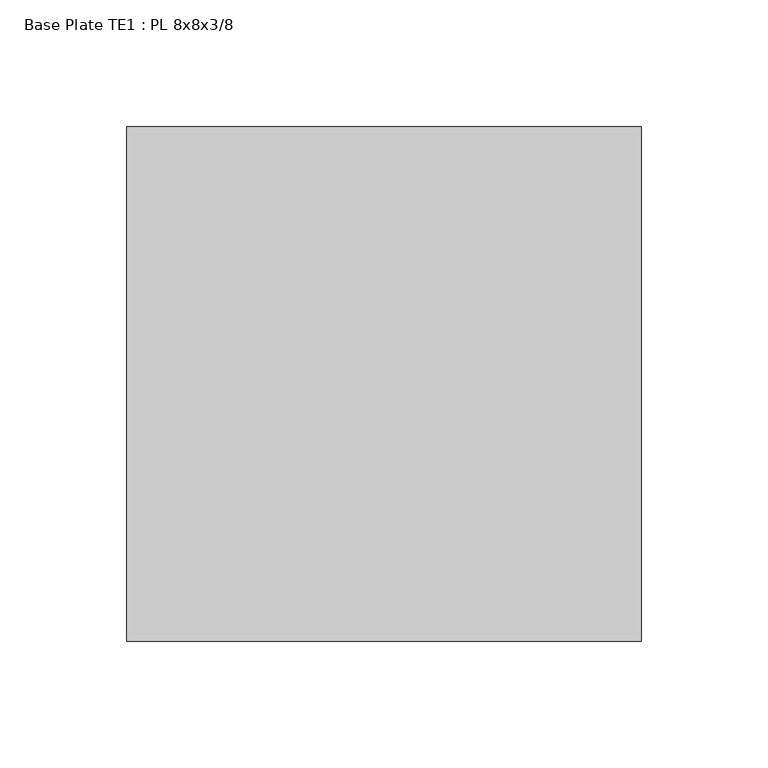
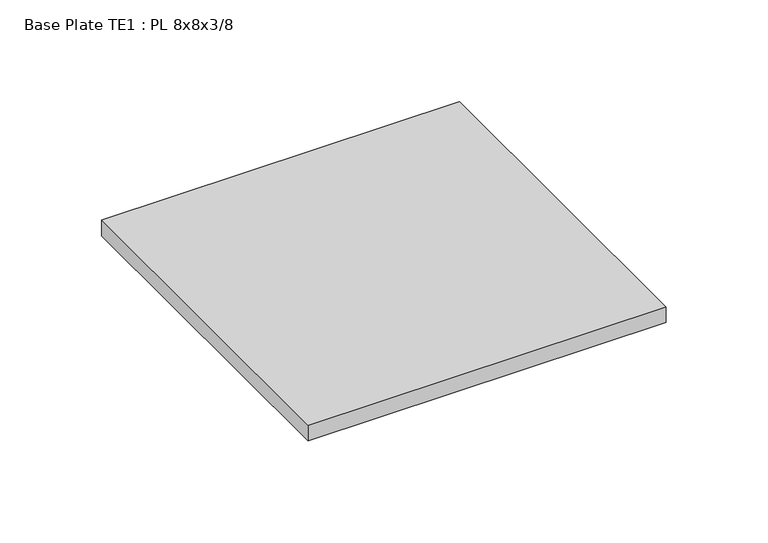
"""IFC4 building model written with IfcOpenShell, lengths in millimetres: proxy geometry, Base Plate TE1 : PL 8x8x3/8."""

from ifc_helpers import new_model, si_unit, frame, origin, place, context, project, spatial, polyline, outline, extrude, source, transform, mapped, element, save


def base_plate_te1_pl_8x8x3_8_a06680a7(model_context):
    return source(origin(), model_context, "Body", "SweptSolid", [
        extrude(outline(polyline([(590318.6599233, -532779.0413841), (590318.6599233, -532982.2413841), (590115.4599233, -532982.2413841), (590115.4599233, -532779.0413841), (590318.6599233, -532779.0413841)])), frame((0.0, 0.0, 19.05), z_axis=(0.0, 0.0, 1.0), x_axis=(1.0, 0.0, 0.0)), (0.0, 0.0, 1.0), 9.525),
    ])


if __name__ == "__main__":
    model = new_model("IFC4")
    model_context = context("Model", 3, world=origin())
    ifc_project = project(units=[si_unit("LENGTHUNIT", "METRE", prefix="MILLI")], contexts=[model_context])
    site = spatial("IfcSite", under=ifc_project)
    building = spatial("IfcBuilding", under=site)
    placement = place(None, origin())
    base_plate_te1_pl_8x8x3_8_shape = base_plate_te1_pl_8x8x3_8_a06680a7(model_context)
    element("IfcBuildingElementProxy", 1, Name="Base Plate TE1 : PL 8x8x3/8", ObjectType="Base Plate TE1 : PL 8x8x3/8", at=placement, inside=building, context=model_context, shape_type="MappedRepresentation", body=[
        mapped(base_plate_te1_pl_8x8x3_8_shape, transform((0.0, 0.0, 0.0), x_axis=(1.0, 0.0, 0.0), y_axis=(0.0, 1.0, 0.0), z_axis=(0.0, 0.0, 1.0))),
    ])
    save(model, "model.ifc")

# Revit data of these elements
# Element 1 (IfcBuildingElementProxy, "Base Plate TE1 : PL 8x8x3/8")
#   Materials on its faces: "GALV. STL BASE PLATE"
# Materials
#   "GALV. STL BASE PLATE": class "Generic", colour RGB 211 211 207, transparency 0, Cost = 0
